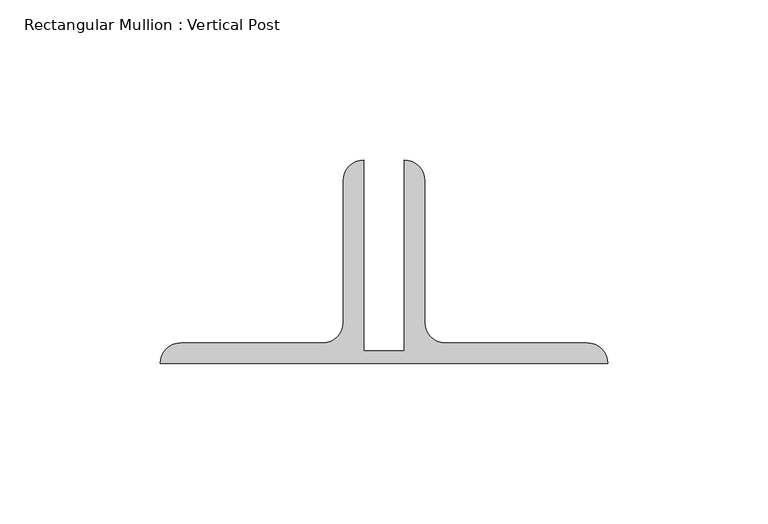
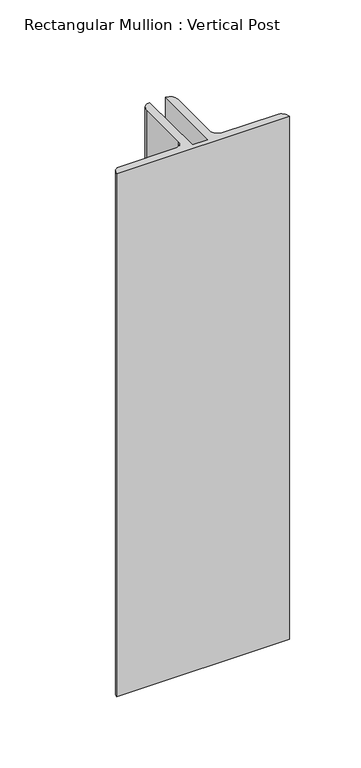
"""IFC4 building model written with IfcOpenShell, lengths in millimetres: member geometry, Rectangular Mullion : Vertical Post."""

import ifcopenshell
import ifcopenshell.guid

model = None  # the IFC model being written
_history = None  # IfcOwnerHistory: only IFC2X3 demands one
_inside = {}  # id of a spatial element -> (the spatial element, [elements in it])
_under = {}  # id of a project, library or spatial element -> (it, [spatial elements below it])
_declared = {}  # id of a project -> (the project, [libraries it declares])
_typed = {}  # id of a type object -> (the type object, [elements of that type])
_made_of = {}  # id of a material, layer set ... -> (it, [elements and type objects made of it])


def new_model(schema):
    """Start an empty IFC model of exactly this schema.

    Asked for "IFC4X3", IfcOpenShell would pick the latest addendum, in which some entities
    have other attributes; the version numbers below select the first issue.
    IFC2X3 requires an IfcOwnerHistory on every rooted entity: one is made here for all.
    """
    global model, _history
    if schema == "IFC4X3":
        model = ifcopenshell.file(schema_version=(4, 3, 0, 0))
    else:
        model = ifcopenshell.file(schema=schema)
    _inside.clear()
    _under.clear()
    _declared.clear()
    _typed.clear()
    _made_of.clear()
    _history = None
    if model.schema == "IFC2X3":
        org = make("IfcOrganization", Name="unknown")
        user = make(
            "IfcPersonAndOrganization",
            ThePerson=make("IfcPerson", FamilyName="unknown"),
            TheOrganization=org,
        )
        app = make(
            "IfcApplication",
            ApplicationDeveloper=org,
            Version="unknown",
            ApplicationFullName="unknown",
            ApplicationIdentifier="unknown",
        )
        _history = make(
            "IfcOwnerHistory",
            OwningUser=user,
            OwningApplication=app,
            ChangeAction="ADDED",
            CreationDate=0,
        )
    return model


def make(cls, **values):
    """One entity of the class cls with the attributes given. An attribute that is None is left unset."""
    return model.create_entity(
        cls, **{name: value for name, value in values.items() if value is not None}
    )


def rooted(cls, **values):
    """An entity with a GlobalId (a new one), such as an element, a storey or a relation."""
    return make(cls, GlobalId=ifcopenshell.guid.new(), OwnerHistory=_history, **values)


def si_unit(unit_type, name, prefix=None):
    """IfcSIUnit, for example si_unit("LENGTHUNIT", "METRE", prefix="MILLI")."""
    return make("IfcSIUnit", UnitType=unit_type, Prefix=prefix, Name=name)


def assignment(units):
    """IfcUnitAssignment: the units of a project."""
    return None if units is None else make("IfcUnitAssignment", Units=units)


def point(xyz):
    """IfcCartesianPoint."""
    return None if xyz is None else make("IfcCartesianPoint", Coordinates=xyz)


def direction(xyz):
    """IfcDirection."""
    return None if xyz is None else make("IfcDirection", DirectionRatios=xyz)


def frame(location, z_axis=None, x_axis=None):
    """IfcAxis2Placement3D, a coordinate frame: its origin and axes. An axis left out is left unset."""
    return make(
        "IfcAxis2Placement3D",
        Location=point(location),
        Axis=direction(z_axis),
        RefDirection=direction(x_axis),
    )


def frame_2d(location, x_axis=None):
    """IfcAxis2Placement2D, a coordinate frame in the plane: its origin and x axis."""
    return make(
        "IfcAxis2Placement2D", Location=point(location), RefDirection=direction(x_axis)
    )


def origin():
    """The frame at (0, 0, 0) with its axes left unset."""
    return frame((0.0, 0.0, 0.0))


def place(relative_to, where):
    """IfcLocalPlacement: puts the frame where relative to a parent placement (None: the world)."""
    return make(
        "IfcLocalPlacement", PlacementRelTo=relative_to, RelativePlacement=where
    )


def context(
    kind, dimensions, precision=None, world=None, true_north=None, identifier=None
):
    """IfcGeometricRepresentationContext, for example the 3D "Model" context."""
    return make(
        "IfcGeometricRepresentationContext",
        ContextIdentifier=identifier,
        ContextType=kind,
        CoordinateSpaceDimension=dimensions,
        Precision=precision,
        WorldCoordinateSystem=world,
        TrueNorth=true_north,
    )


def project(units=None, contexts=None):
    """IfcProject with its units and contexts."""
    return rooted(
        "IfcProject",
        Name="project",
        RepresentationContexts=contexts,
        UnitsInContext=assignment(units),
    )


def spatial(cls, under=None, at=None, **own):
    """A site, building, storey or space (cls), placed at a placement, below another one or the project."""
    s = rooted(cls, ObjectPlacement=at, **own)
    if under is not None:
        _under.setdefault(under.id(), (under, []))[1].append(s)
    return s


def polyline(points):
    """IfcPolyline through the points."""
    return make("IfcPolyline", Points=[point(p) for p in points])


def circle_curve(where, radius):
    """IfcCircle in the frame where."""
    return make("IfcCircle", Position=where, Radius=radius)


def trimmed(basis, trim1, trim2, sense, master):
    """IfcTrimmedCurve: the piece of a basis curve between two trims."""
    return make(
        "IfcTrimmedCurve",
        BasisCurve=basis,
        Trim1=trim1,
        Trim2=trim2,
        SenseAgreement=sense,
        MasterRepresentation=master,
    )


def segment(curve, same_sense, transition):
    """IfcCompositeCurveSegment."""
    return make(
        "IfcCompositeCurveSegment",
        Transition=transition,
        SameSense=same_sense,
        ParentCurve=curve,
    )


def composite_curve(segments, self_intersect=None):
    """IfcCompositeCurve: segments joined end to end."""
    return make("IfcCompositeCurve", Segments=segments, SelfIntersect=self_intersect)


def outline(outer, holes=None, kind="AREA"):
    """IfcArbitraryClosedProfileDef: a profile drawn as a closed curve; with holes, ...WithVoids."""
    if holes is None:
        return make("IfcArbitraryClosedProfileDef", ProfileType=kind, OuterCurve=outer)
    return make(
        "IfcArbitraryProfileDefWithVoids",
        ProfileType=kind,
        OuterCurve=outer,
        InnerCurves=holes,
    )


def extrude(swept, where, along, depth):
    """IfcExtrudedAreaSolid: the profile swept, set in the frame where, extruded along a direction by depth."""
    return make(
        "IfcExtrudedAreaSolid",
        SweptArea=swept,
        Position=where,
        ExtrudedDirection=direction(along),
        Depth=depth,
    )


def shape(context_of_items, identifier, shape_type, items):
    """IfcShapeRepresentation: the items that make up one representation, for example the "Body"."""
    return make(
        "IfcShapeRepresentation",
        ContextOfItems=context_of_items,
        RepresentationIdentifier=identifier,
        RepresentationType=shape_type,
        Items=items,
    )


def source(mapping_origin, context_of_items, identifier, shape_type, items):
    """IfcRepresentationMap: a shape defined once, which mapped items show again and again."""
    return make(
        "IfcRepresentationMap",
        MappingOrigin=mapping_origin,
        MappedRepresentation=shape(context_of_items, identifier, shape_type, items),
    )


def transform(
    local_origin,
    x_axis=None,
    y_axis=None,
    z_axis=None,
    scale=None,
    scale2=None,
    scale3=None,
    uniform=True,
):
    """IfcCartesianTransformationOperator3D, or its non-uniform kind. x_axis, y_axis, z_axis: its Axis1, 2, 3."""
    if uniform:
        return make(
            "IfcCartesianTransformationOperator3D",
            Axis1=direction(x_axis),
            Axis2=direction(y_axis),
            LocalOrigin=point(local_origin),
            Scale=scale,
            Axis3=direction(z_axis),
        )
    return make(
        "IfcCartesianTransformationOperator3DnonUniform",
        Axis1=direction(x_axis),
        Axis2=direction(y_axis),
        LocalOrigin=point(local_origin),
        Scale=scale,
        Axis3=direction(z_axis),
        Scale2=scale2,
        Scale3=scale3,
    )


def mapped(mapping_source, mapping_target):
    """IfcMappedItem: shows the shape of a source again, moved by a transform."""
    return make(
        "IfcMappedItem", MappingSource=mapping_source, MappingTarget=mapping_target
    )


def made_of(thing, what):
    """Note that an element or type object is made of a material, layer set ...; save() writes the relation."""
    if what is not None:
        _made_of.setdefault(what.id(), (what, []))[1].append(thing)
    return thing


def element(
    cls,
    number,
    at=None,
    inside=None,
    cuts=None,
    type_object=None,
    material=None,
    context=None,
    identifier="Body",
    shape_type=None,
    held_by="IfcProductDefinitionShape",
    body=None,
    shapes=None,
    **own,
):
    """One element of the class cls, such as IfcWall. Its Tag is "e" and its number.

    at: its placement. inside: the storey or other place that contains it. cuts: it is an
    opening in that element (IfcRelVoidsElement). A single representation is given by context,
    identifier, shape_type and body (its items); several are given by shapes. held_by: the class
    of the entity that holds the representations. save() writes the other relations.
    """
    e = rooted(cls, Tag="e%d" % number, ObjectPlacement=at, **own)
    if body is not None:
        shapes = [shape(context, identifier, shape_type, body)]
    if shapes is not None:
        e.Representation = make(held_by, Representations=shapes)
    if inside is not None:
        _inside.setdefault(inside.id(), (inside, []))[1].append(e)
    if cuts is not None:
        rooted(
            "IfcRelVoidsElement", RelatingBuildingElement=cuts, RelatedOpeningElement=e
        )
    if type_object is not None:
        _typed.setdefault(type_object.id(), (type_object, []))[1].append(e)
    return made_of(e, material)


def aggregate(whole, parts):
    """IfcRelAggregates: a whole, such as a stair, and the parts it consists of."""
    return rooted("IfcRelAggregates", RelatingObject=whole, RelatedObjects=parts)


def save(model, path):
    """Write the relations noted so far, then the file.

    IfcRelAggregates (storeys below a building ...), IfcRelContainedInSpatialStructure (elements
    in a storey), IfcRelDefinesByType, IfcRelAssociatesMaterial and IfcRelDeclares: one each for
    every whole, place, type object, material and project.
    """
    for whole, parts in _under.values():
        aggregate(whole, parts)
    for where, things in _inside.values():
        rooted(
            "IfcRelContainedInSpatialStructure",
            RelatedElements=things,
            RelatingStructure=where,
        )
    for kind, things in _typed.values():
        rooted("IfcRelDefinesByType", RelatedObjects=things, RelatingType=kind)
    for what, things in _made_of.values():
        rooted("IfcRelAssociatesMaterial", RelatedObjects=things, RelatingMaterial=what)
    for by, libraries in _declared.values():
        rooted("IfcRelDeclares", RelatingContext=by, RelatedDefinitions=libraries)
    model.write(path)


def rectangular_mullion_vertical_post_4fcf061c(model_context):
    return source(origin(), model_context, "Body", "SweptSolid", [
        extrude(outline(composite_curve([segment(polyline([(-6.35, 22.9145205), (6.35, 22.9145205), (6.35, 82.55)]), True, "CONTINUOUS"), segment(trimmed(circle_curve(frame_2d((6.35, 76.2)), 6.35), [point((6.35, 82.55))], [point((12.7, 76.2))], False, "CARTESIAN"), True, "CONTINUOUS"), segment(polyline([(12.7, 76.2), (12.7, 31.75)]), True, "CONTINUOUS"), segment(trimmed(circle_curve(frame_2d((19.05, 31.75)), 6.35), [point((12.7, 31.75))], [point((19.05, 25.4))], True, "CARTESIAN"), True, "CONTINUOUS"), segment(polyline([(19.05, 25.4), (63.5, 25.4)]), True, "CONTINUOUS"), segment(trimmed(circle_curve(frame_2d((63.5, 19.05)), 6.35), [point((63.5, 25.4))], [point((69.85, 19.05))], False, "CARTESIAN"), True, "CONTINUOUS"), segment(polyline([(69.85, 19.05), (-69.85, 19.05)]), True, "CONTINUOUS"), segment(trimmed(circle_curve(frame_2d((-63.5, 19.05)), 6.35), [point((-69.85, 19.05))], [point((-63.5, 25.4))], False, "CARTESIAN"), True, "CONTINUOUS"), segment(polyline([(-63.5, 25.4), (-19.05, 25.4)]), True, "CONTINUOUS"), segment(trimmed(circle_curve(frame_2d((-19.05, 31.75)), 6.35), [point((-19.05, 25.4))], [point((-12.7, 31.75))], True, "CARTESIAN"), True, "CONTINUOUS"), segment(polyline([(-12.7, 31.75), (-12.7, 76.2)]), True, "CONTINUOUS"), segment(trimmed(circle_curve(frame_2d((-6.35, 76.2)), 6.35), [point((-12.7, 76.2))], [point((-6.35, 82.55))], False, "CARTESIAN"), True, "CONTINUOUS"), segment(polyline([(-6.35, 82.55), (-6.35, 22.9145205)]), True, "CONTINUOUS")], self_intersect=False)), frame((0.0, 0.0, -446.7663052), z_axis=(0.0, 0.0, 1.0), x_axis=(1.0, 0.0, 0.0)), (0.0, 0.0, 1.0), 446.7663052),
    ])


if __name__ == "__main__":
    model = new_model("IFC4")
    model_context = context("Model", 3, world=origin())
    ifc_project = project(units=[si_unit("LENGTHUNIT", "METRE", prefix="MILLI")], contexts=[model_context])
    site = spatial("IfcSite", under=ifc_project)
    building = spatial("IfcBuilding", under=site)
    placement = place(None, origin())
    rectangular_mullion_vertical_post_shape = rectangular_mullion_vertical_post_4fcf061c(model_context)
    element("IfcMember", 1, ObjectType="Rectangular Mullion : Vertical Post", at=placement, inside=building, context=model_context, shape_type="MappedRepresentation", body=[
        mapped(rectangular_mullion_vertical_post_shape, transform((0.0, 0.0, 0.0), x_axis=(1.0, 0.0, 0.0), y_axis=(0.0, 1.0, 0.0), z_axis=(0.0, 0.0, 1.0))),
    ])
    save(model, "model.ifc")

# Revit data of these elements
# Type "Rectangular Mullion : Vertical Post"
#   built-in parameter 1007351 = -0.0625 (stored number, unit not read)
#   built-in parameter 1007322 = 0.0126789 (stored number, unit not read)
#   built-in parameter 1007321 = 0.229167 (stored number, unit not read)
#   built-in parameter 1007320 = 0.229167 (stored number, unit not read)
# Element 1 (IfcMember, "Rectangular Mullion : Vertical Post")
#   Materials on its faces: "GATE POST: (2) BACK/BACK GALVANIZED ANGLES"
# Materials
#   "GATE POST: (2) BACK/BACK GALVANIZED ANGLES": class "Unassigned", colour RGB 211 211 211, transparency 0, Cost = 0
